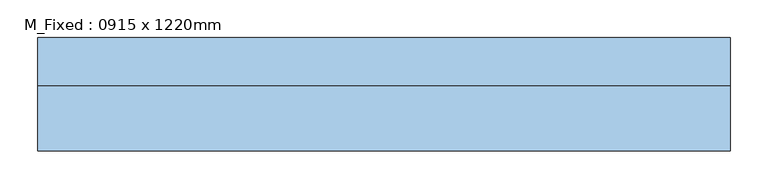
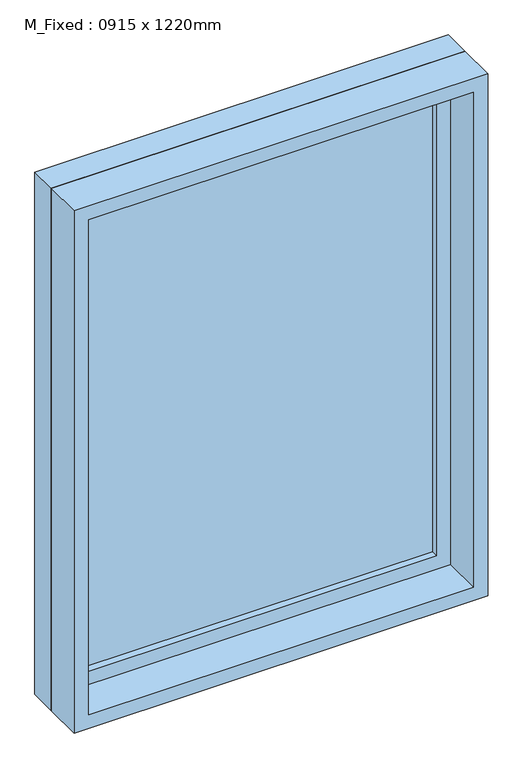
"""IFC4 building model written with IfcOpenShell, lengths in millimetres: window geometry, M_Fixed : 0915 x 1220mm."""

from ifc_helpers import new_model, si_unit, frame, origin, place, context, project, spatial, polyline, outline, extrude, source, transform, mapped, element, save


def m_fixed_0915_x_1220mm_873aa0e2(model_context):
    return source(origin(), model_context, "Body", "SweptSolid", [
        extrude(outline(polyline([(-394.5, 53.0), (394.5, 53.0), (394.5, 41.0), (-394.5, 41.0), (-394.5, 53.0)])), frame((0.0, 0.0, 978.0), z_axis=(0.0, 0.0, 1.0), x_axis=(1.0, 0.0, 0.0)), (0.0, 0.0, 1.0), 1094.0),
        extrude(outline(polyline([(2116.0, -438.5), (934.0, -438.5), (934.0, 438.5), (2116.0, 438.5), (2116.0, -438.5)]), holes=[polyline([(2072.0, -394.5), (2072.0, 394.5), (978.0, 394.5), (978.0, -394.5), (2072.0, -394.5)])]), frame((0.0, 25.0, 0.0), z_axis=(0.0, 1.0, 0.0), x_axis=(0.0, 0.0, 1.0)), (0.0, 0.0, 1.0), 44.0),
        extrude(outline(polyline([(2135.0, -457.5), (915.0, -457.5), (915.0, 457.5), (2135.0, 457.5), (2135.0, -457.5)]), holes=[polyline([(2116.0, -438.5), (2116.0, 438.5), (934.0, 438.5), (934.0, -438.5), (2116.0, -438.5)])]), frame((0.0, 25.0, 0.0), z_axis=(0.0, 1.0, 0.0), x_axis=(0.0, 0.0, 1.0)), (0.0, 0.0, 1.0), 63.0),
        extrude(outline(polyline([(2135.0, -457.5), (915.0, -457.5), (915.0, 457.5), (2135.0, 457.5), (2135.0, -457.5)]), holes=[polyline([(2103.0, -425.5), (2103.0, 425.5), (947.0, 425.5), (947.0, -425.5), (2103.0, -425.5)])]), frame((0.0, -62.0, 0.0), z_axis=(0.0, 1.0, 0.0), x_axis=(0.0, 0.0, 1.0)), (0.0, 0.0, 1.0), 87.0),
    ])


if __name__ == "__main__":
    model = new_model("IFC4")
    model_context = context("Model", 3, world=origin())
    ifc_project = project(units=[si_unit("LENGTHUNIT", "METRE", prefix="MILLI")], contexts=[model_context])
    site = spatial("IfcSite", under=ifc_project)
    building = spatial("IfcBuilding", under=site)
    placement = place(None, origin())
    m_fixed_0915_x_1220mm_shape = m_fixed_0915_x_1220mm_873aa0e2(model_context)
    element("IfcWindow", 1, ObjectType="M_Fixed : 0915 x 1220mm", at=placement, inside=building, context=model_context, shape_type="MappedRepresentation", body=[
        mapped(m_fixed_0915_x_1220mm_shape, transform((0.0, 0.0, 0.0), x_axis=(1.0, 0.0, 0.0), y_axis=(0.0, 1.0, 0.0), z_axis=(0.0, 0.0, 1.0))),
    ])
    save(model, "model.ifc")

# Revit data of these elements
# Type "M_Fixed : 0915 x 1220mm"
#   Type Mark = "15"
#   Height = 1.22 m
#   Default Sill Height = 0.915 m
#   Width = 0.915 m
#   Window Inset = 0.019 m
#   Frame Exterior Material = Sash
#   Frame Interior Material = Sash
#   Glass Pane Material = Glass
#   Sash = Sash
#   Wall Closure = (empty or 0)
# Element 1 (IfcWindow, "M_Fixed : 0915 x 1220mm")
#   Materials on its faces: "Sash", "Glass"
# Materials
#   "Sash": class "Wood", colour RGB 136 99 55, transparency 0
#   "Glass": class "Glass", colour RGB 218 227 224, transparency 0.85, Description = "Soda Lime Glass", Cost = 0
